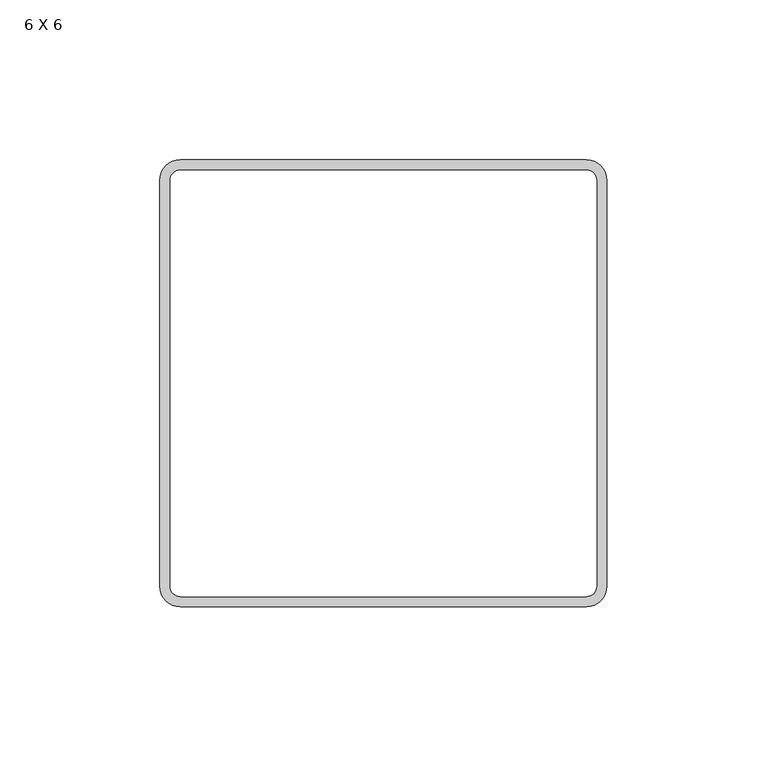
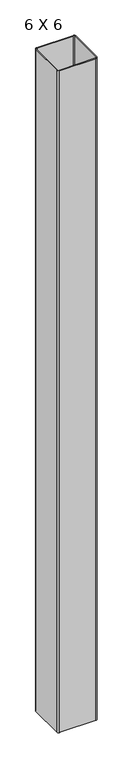
"""IFC4 building model written with IfcOpenShell, lengths in millimetres: column geometry, Structural_Column-Trex-Deck_Support_Post : 6 X 6."""

from ifc_helpers import new_model, si_unit, point, frame_2d, origin, origin_with_axes, place, context, project, spatial, polyline, circle_curve, trimmed, segment, composite_curve, outline, extrude, source, transform, mapped, element, save


def column_6_x_6_d1425c31(model_context):
    return source(origin(), model_context, "Body", "SweptSolid", [
        extrude(outline(composite_curve([segment(polyline([(-63.5, 69.85), (63.5, 69.85)]), True, "CONTINUOUS"), segment(trimmed(circle_curve(frame_2d((63.5, 63.5)), 6.35), [point((63.5, 69.85))], [point((69.85, 63.5))], False, "CARTESIAN"), True, "CONTINUOUS"), segment(polyline([(69.85, 63.5), (69.85, -63.5)]), True, "CONTINUOUS"), segment(trimmed(circle_curve(frame_2d((63.5, -63.5)), 6.35), [point((69.85, -63.5))], [point((63.5, -69.85))], False, "CARTESIAN"), True, "CONTINUOUS"), segment(polyline([(63.5, -69.85), (-63.5, -69.85)]), True, "CONTINUOUS"), segment(trimmed(circle_curve(frame_2d((-63.5, -63.5)), 6.35), [point((-63.5, -69.85))], [point((-69.85, -63.5))], False, "CARTESIAN"), True, "CONTINUOUS"), segment(polyline([(-69.85, -63.5), (-69.85, 63.5)]), True, "CONTINUOUS"), segment(trimmed(circle_curve(frame_2d((-63.5, 63.5)), 6.35), [point((-69.85, 63.5))], [point((-63.5, 69.85))], False, "CARTESIAN"), True, "CONTINUOUS")], self_intersect=False), holes=[composite_curve([segment(trimmed(circle_curve(frame_2d((-63.5, 63.5)), 3.175), [point((-63.5, 66.675))], [point((-66.675, 63.5))], True, "CARTESIAN"), True, "CONTINUOUS"), segment(polyline([(-66.675, 63.5), (-66.675, -63.5)]), True, "CONTINUOUS"), segment(trimmed(circle_curve(frame_2d((-63.5, -63.5)), 3.175), [point((-66.675, -63.5))], [point((-63.5, -66.675))], True, "CARTESIAN"), True, "CONTINUOUS"), segment(polyline([(-63.5, -66.675), (63.5, -66.675)]), True, "CONTINUOUS"), segment(trimmed(circle_curve(frame_2d((63.5, -63.5)), 3.175), [point((63.5, -66.675))], [point((66.675, -63.5))], True, "CARTESIAN"), True, "CONTINUOUS"), segment(polyline([(66.675, -63.5), (66.675, 63.5)]), True, "CONTINUOUS"), segment(trimmed(circle_curve(frame_2d((63.5, 63.5)), 3.175), [point((66.675, 63.5))], [point((63.5, 66.675))], True, "CARTESIAN"), True, "CONTINUOUS"), segment(polyline([(63.5, 66.675), (-63.5, 66.675)]), True, "CONTINUOUS")], self_intersect=False)]), origin_with_axes(), (0.0, 0.0, 1.0), 2436.8125),
    ])


if __name__ == "__main__":
    model = new_model("IFC4")
    model_context = context("Model", 3, world=origin())
    ifc_project = project(units=[si_unit("LENGTHUNIT", "METRE", prefix="MILLI")], contexts=[model_context])
    site = spatial("IfcSite", under=ifc_project)
    building = spatial("IfcBuilding", under=site)
    placement = place(None, origin())
    column_6_x_6_shape = column_6_x_6_d1425c31(model_context)
    element("IfcColumn", 1, ObjectType="Structural_Column-Trex-Deck_Support_Post : 6 X 6", at=placement, inside=building, context=model_context, shape_type="MappedRepresentation", body=[
        mapped(column_6_x_6_shape, transform((0.0, 0.0, 0.0), x_axis=(1.0, 0.0, 0.0), y_axis=(0.0, 1.0, 0.0), z_axis=(0.0, 0.0, 1.0))),
    ])
    save(model, "model.ifc")

# Revit data of these elements
# Type "Structural_Column-Trex-Deck_Support_Post : 6 X 6"
#   URL = "www.trex.com"
#   Product Page URL = "http://www.trex.com/products/deck-framing-drainage/elevations/"
#   Product Name = "Trex Elevations® Support Post"
#   Product Documentation Link = "http://www.trex.com/trex/groups/content/@mktgtechsvc/documents/document/trexmd_010019.pdf"
#   Model = "Support Post"
#   Material = ""
#   Manufacturer = "Trex®"
#   Description = "Steel Deck Framing"
#   Width = 0' - 5 1/2"
#   Thickness = 0' - 0 1/8"
#   Depth = 0' - 5 1/2"
#   Detail Component = yes
#   Structural Material [instance default] = Metal Joists - Trex - Elevations® Steel Deck Framing - 2x8
# Element 1 (IfcColumn, "Structural_Column-Trex-Deck_Support_Post : 6 X 6")
#   Structural Material = ALL 5.5"X5.5" GLULAM COLUMNS - ARCHITECTURAL APPEARANCE - FINISH ALL 4 SIDES - STAIN T.B.D.
#   Materials on its faces: "ALL 5.5\"X5.5\" GLULAM COLUMNS - ARCHITECTURAL APPEARANCE - FINISH ALL 4 SIDES - STAIN T.B.D."
# Materials
#   "Metal Joists - Trex - Elevations® Steel Deck Framing - 2x8": class "Wood", colour RGB 114 102 88, transparency 0, Keynote = "05 42 16", Model = "Trex Elevations® Steel Deck Framing", Manufacturer = "Trex", URL = "http://www.trex.com/", Description = "2x8 Trex Elevations® Steel Deck Framing", Cost = 0
#   "ALL 5.5\"X5.5\" GLULAM COLUMNS - ARCHITECTURAL APPEARANCE - FINISH ALL 4 SIDES - STAIN T.B.D.": class "Wood", colour RGB 234 198 147, transparency 0, Description = "Pinus Echinata", Cost = 0
